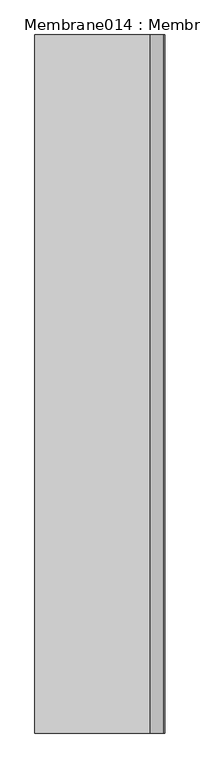
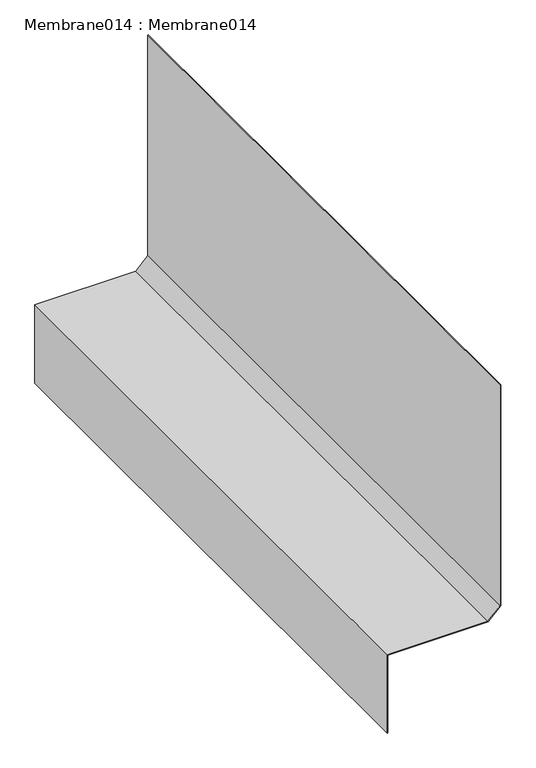
"""IFC4 building model written with IfcOpenShell, lengths in millimetres: proxy geometry, Membrane014 : Membrane014."""

from ifc_helpers import new_model, si_unit, frame, origin, place, context, project, spatial, polyline, outline, extrude, source, transform, mapped, element, save


def membrane014_membrane014_b0364b1d(model_context):
    return source(origin(), model_context, "Body", "SweptSolid", [
        extrude(outline(polyline([(33390.8554688, -9663.9882813), (32626.9430944, -9663.9882813), (32586.6386719, -9703.8524464), (32586.6386719, -10033.7987014), (32314.8961275, -10033.7987014), (32314.8961275, -10031.7987014), (32584.6386719, -10031.7987014), (32584.6386719, -9703.0175781), (32626.1210938, -9661.9882813), (33390.8554688, -9661.9882813), (33390.8554688, -9663.9882813)])), frame((0.0, 7982.1531721, 0.0), z_axis=(0.0, 1.0, 0.0), x_axis=(0.0, 0.0, 1.0)), (0.0, 0.0, 1.0), 2000.0),
    ])


if __name__ == "__main__":
    model = new_model("IFC4")
    model_context = context("Model", 3, world=origin())
    ifc_project = project(units=[si_unit("LENGTHUNIT", "METRE", prefix="MILLI")], contexts=[model_context])
    site = spatial("IfcSite", under=ifc_project)
    building = spatial("IfcBuilding", under=site)
    placement = place(None, origin())
    membrane014_membrane014_shape = membrane014_membrane014_b0364b1d(model_context)
    element("IfcBuildingElementProxy", 1, Name="Membrane014 : Membrane014", ObjectType="Membrane014 : Membrane014", at=placement, inside=building, context=model_context, shape_type="MappedRepresentation", body=[
        mapped(membrane014_membrane014_shape, transform((0.0, 0.0, 0.0), x_axis=(1.0, 0.0, 0.0), y_axis=(0.0, 1.0, 0.0), z_axis=(0.0, 0.0, 1.0))),
    ])
    save(model, "model.ifc")

# Revit data of these elements
# Type "Membrane014 : Membrane014"
#   NameOverride = "Membrane014"
# Element 1 (IfcBuildingElementProxy, "Membrane014 : Membrane014")
#   Materials on its faces: "BITUMINOUS MEMBRANE - TBD"
# Materials
#   "BITUMINOUS MEMBRANE - TBD": class "Unassigned", colour RGB 0 171 31, transparency 0
